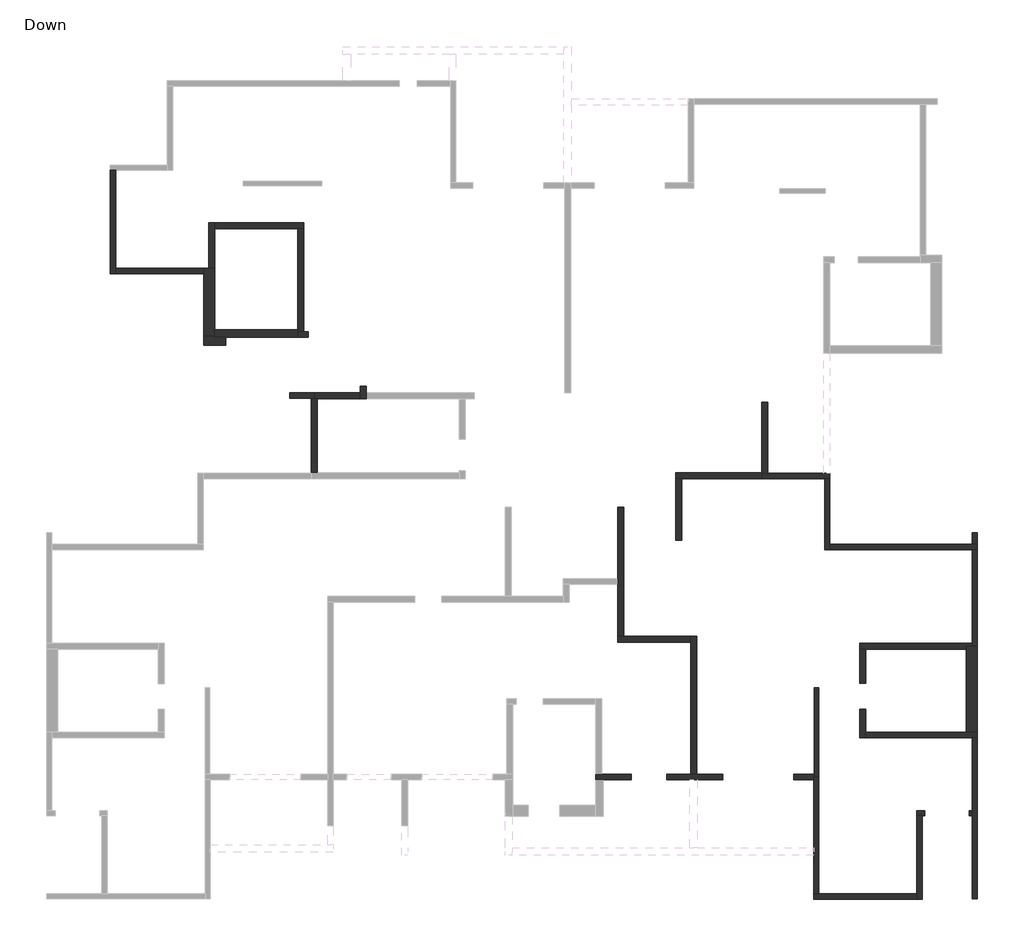
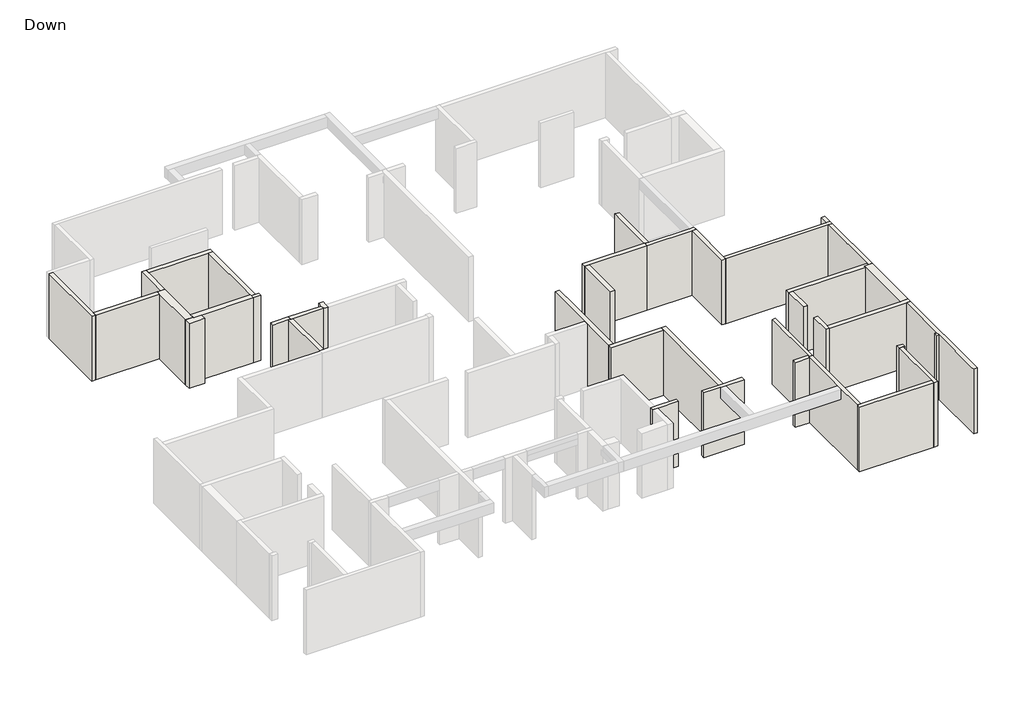
# One storey, part 2 of 3: 39 walls.
"""IFC4 building model written with IfcOpenShell, lengths in millimetres."""

from ifc_helpers import new_model, si_unit, origin, origin_with_axes, place, context, project, spatial, polyline, outline, extrude, faceted_brep, element, save

model = new_model("IFC4")

# Units and contexts
model_context = context("Model", 3, world=origin())
ifc_project = project(units=[si_unit("LENGTHUNIT", "METRE", prefix="MILLI")], contexts=[model_context])

# Site, building, storey
site = spatial("IfcSite", under=ifc_project)
building = spatial("IfcBuilding", under=site)
storey = spatial("IfcBuildingStorey", under=building, Name="Down", Elevation=0.0)

# Walls
placement = place(None, origin())
element("IfcWall", 1, ObjectType="15", at=placement, inside=storey, context=model_context, shape_type="Brep", body=[
    faceted_brep([(7365.3434642, -11434.051338, 0.0), (7365.3434642, -8419.051338, 0.0), (7365.3434642, -8419.051338, 3000.0), (7365.3434642, -8419.051338, 3200.0), (7365.3434642, -11434.051338, 3200.0), (7215.3434642, -11434.051338, 0.0), (7215.3434642, -11434.051338, 3200.0), (7215.3434642, -11344.051338, 3200.0), (7215.3434642, -8419.051338, 3200.0), (7215.3434642, -8419.051338, 3000.0), (7215.3434642, -8419.051338, 0.0), (7215.3434642, -11344.051338, 0.0)], [[[0, 1, 2, 3, 4]], [[5, 6, 7, 8, 9, 10, 11]], [[1, 0, 5, 11, 10]], [[3, 2, 1, 10, 9, 8]], [[4, 3, 8, 7, 6]], [[0, 4, 6, 5]]]),
])
element("IfcWall", 2, ObjectType="18", at=placement, inside=storey, context=model_context, shape_type="Brep", body=[
    faceted_brep([(-16547.4366188, 9037.0772927, 0.0), (-16547.4366188, 5556.9611102, 0.0), (-16547.4366188, 5556.9611102, 3200.0), (-16547.4366188, 9037.0772927, 3200.0), (-16367.4366188, 9037.0772927, 0.0), (-16367.4366188, 9037.0772927, 3000.0), (-16367.4366188, 9037.0772927, 3200.0), (-16367.4366188, 5736.9611102, 3200.0), (-16367.4366188, 5556.9611102, 3200.0), (-16367.4366188, 5556.9611102, 0.0), (-16367.4366188, 5736.9611102, 0.0)], [[[0, 1, 2, 3]], [[4, 5, 6, 7, 8, 9, 10]], [[1, 0, 4, 10, 9]], [[3, 2, 8, 7, 6]], [[0, 3, 6, 5, 4]], [[2, 1, 9, 8]]]),
])
element("IfcWall", 3, ObjectType="18", at=placement, inside=storey, context=model_context, shape_type="Brep", body=[
    faceted_brep([(-16367.4366188, 5556.9611102, 0.0), (-13386.7312246, 5556.9611102, 0.0), (-13386.7312246, 5556.9611102, 3200.0), (-16367.4366188, 5556.9611102, 3200.0), (-16367.4366188, 5736.9611102, 0.0), (-16367.4366188, 5736.9611102, 3000.0), (-16367.4366188, 5736.9611102, 3200.0), (-13386.7312246, 5736.9611102, 3200.0), (-13386.7312246, 5736.9611102, 0.0)], [[[0, 1, 2, 3]], [[4, 5, 6, 7, 8]], [[1, 0, 4, 8]], [[3, 2, 7, 6]], [[0, 3, 6, 5, 4]], [[2, 1, 8, 7]]]),
])
element("IfcWall", 4, ObjectType="18", at=placement, inside=storey, context=model_context, shape_type="Brep", body=[
    faceted_brep([(-10217.2125524, 3416.4548861, 0.0), (-9872.2125524, 3416.4548861, 0.0), (-9872.2125524, 3416.4548861, 3000.0), (-9872.2125524, 3416.4548861, 3200.0), (-10217.2125524, 3416.4548861, 3200.0), (-10217.2125524, 3596.4548861, 0.0), (-10217.2125524, 3596.4548861, 3200.0), (-10017.2125524, 3596.4548861, 3200.0), (-9872.2125524, 3596.4548861, 3200.0), (-9872.2125524, 3596.4548861, 3000.0), (-9872.2125524, 3596.4548861, 0.0), (-10017.2125524, 3596.4548861, 0.0)], [[[0, 1, 2, 3, 4]], [[5, 6, 7, 8, 9, 10, 11]], [[1, 0, 5, 11, 10]], [[3, 2, 1, 10, 9, 8]], [[4, 3, 8, 7, 6]], [[0, 4, 6, 5]]]),
])
element("IfcWall", 5, ObjectType="18", at=placement, inside=storey, context=model_context, shape_type="Brep", body=[
    faceted_brep([(7735.384958, -1184.051338, 0.0), (5633.824792, -1184.051338, 0.0), (5433.824792, -1184.051338, 0.0), (5433.824792, -1184.051338, 3200.0), (5633.824792, -1184.051338, 3200.0), (7535.1359953, -1184.051338, 3200.0), (7735.384958, -1184.051338, 3200.0), (7735.384958, -1364.051338, 0.0), (7735.384958, -1364.051338, 3200.0), (7555.384958, -1364.051338, 3200.0), (5433.824792, -1364.051338, 3200.0), (5433.824792, -1364.051338, 0.0), (7555.384958, -1364.051338, 0.0)], [[[0, 1, 2, 3, 4, 5, 6]], [[7, 8, 9, 10, 11, 12]], [[2, 1, 0, 7, 12, 11]], [[6, 5, 4, 3, 10, 9, 8]], [[3, 2, 11, 10]], [[0, 6, 8, 7]]]),
])
element("IfcWall", 6, ObjectType="18", at=placement, inside=storey, context=model_context, shape_type="Brep", body=[
    faceted_brep([(7555.384958, -1364.051338, 0.0), (7555.384958, -3764.1011305, 0.0), (7555.384958, -3764.1011305, 3000.0), (7555.384958, -3764.1011305, 3200.0), (7555.384958, -1364.051338, 3200.0), (7555.384958, -1364.051338, 3000.0), (7735.384958, -1364.051338, 0.0), (7735.384958, -1364.051338, 3200.0), (7735.384958, -3584.1011305, 3200.0), (7735.384958, -3764.1011305, 3200.0), (7735.384958, -3764.1011305, 0.0), (7735.384958, -3584.1011305, 0.0)], [[[0, 1, 2, 3, 4, 5]], [[6, 7, 8, 9, 10, 11]], [[1, 0, 6, 11, 10]], [[4, 3, 9, 8, 7]], [[3, 2, 1, 10, 9]], [[0, 5, 4, 7, 6]]]),
])
element("IfcWall", 7, ObjectType="18", at=placement, inside=storey, context=model_context, shape_type="Brep", body=[
    faceted_brep([(7735.384958, -3764.1011305, 0.0), (12534.2065347, -3764.1011305, 0.0), (12714.2065347, -3764.1011305, 0.0), (12714.2065347, -3764.1011305, 3200.0), (12534.2065347, -3764.1011305, 3200.0), (7735.384958, -3764.1011305, 3200.0), (7735.384958, -3584.1011305, 0.0), (7735.384958, -3584.1011305, 3200.0), (12534.2065347, -3584.1011305, 3200.0), (12714.2065347, -3584.1011305, 3200.0), (12714.2065347, -3584.1011305, 0.0), (12534.2065347, -3584.1011305, 0.0)], [[[0, 1, 2, 3, 4, 5]], [[6, 7, 8, 9, 10, 11]], [[2, 1, 0, 6, 11, 10]], [[5, 4, 3, 9, 8, 7]], [[0, 5, 7, 6]], [[3, 2, 10, 9]]]),
])
element("IfcWall", 8, ObjectType="18", at=placement, inside=storey, context=model_context, shape_type="SweptSolid", body=[
    extrude(outline(polyline([(12714.2065347, -3184.4330807), (12714.2065347, -3584.1011305), (12534.2065347, -3584.1011305), (12534.2065347, -3184.4330807), (12714.2065347, -3184.4330807)])), origin_with_axes(), (0.0, 0.0, 1.0), 3200.0),
])
element("IfcWall", 9, ObjectType="18", at=placement, inside=storey, context=model_context, shape_type="Brep", body=[
    faceted_brep([(12534.2065347, -3764.1011305, 0.0), (12534.2065347, -6913.2795537, 0.0), (12534.2065347, -7013.2795537, 0.0), (12534.2065347, -7013.2795537, 3200.0), (12534.2065347, -6913.2795537, 3200.0), (12534.2065347, -3764.1011305, 3200.0), (12534.2065347, -3764.1011305, 3000.0), (12714.2065347, -3764.1011305, 0.0), (12714.2065347, -3764.1011305, 3200.0), (12714.2065347, -7013.2795537, 3200.0), (12714.2065347, -7013.2795537, 0.0)], [[[0, 1, 2, 3, 4, 5, 6]], [[7, 8, 9, 10]], [[2, 1, 0, 7, 10]], [[3, 2, 10, 9]], [[5, 4, 3, 9, 8]], [[0, 6, 5, 8, 7]]]),
])
element("IfcWall", 10, ObjectType="18", at=placement, inside=storey, context=model_context, shape_type="Brep", body=[
    faceted_brep([(12534.2065347, -10113.0471886, 0.0), (12534.2065347, -12564.5160683, 0.0), (12534.2065347, -12744.5160683, 0.0), (12534.2065347, -15545.0637861, 0.0), (12534.2065347, -15545.0637861, 3200.0), (12534.2065347, -15369.5160683, 3200.0), (12534.2065347, -12744.5160683, 3200.0), (12534.2065347, -12564.5160683, 3200.0), (12534.2065347, -10113.0471886, 3200.0), (12534.2065347, -10113.0471886, 3000.0), (12714.2065347, -10113.0471886, 0.0), (12714.2065347, -10113.0471886, 3200.0), (12714.2065347, -15545.0637861, 3200.0), (12714.2065347, -15545.0637861, 0.0)], [[[0, 1, 2, 3, 4, 5, 6, 7, 8, 9]], [[10, 11, 12, 13]], [[3, 2, 1, 0, 10, 13]], [[4, 3, 13, 12]], [[8, 7, 6, 5, 4, 12, 11]], [[0, 9, 8, 11, 10]]]),
])
element("IfcWall", 11, ObjectType="18", at=placement, inside=storey, context=model_context, shape_type="Brep", body=[
    faceted_brep([(12534.2065347, -12564.5160683, 0.0), (12429.6422194, -12564.5160683, 0.0), (12429.6422194, -12564.5160683, 3000.0), (12429.6422194, -12564.5160683, 3200.0), (12534.2065347, -12564.5160683, 3200.0), (12534.2065347, -12564.5160683, 3000.0), (12534.2065347, -12744.5160683, 0.0), (12534.2065347, -12744.5160683, 2980.0), (12534.2065347, -12744.5160683, 3200.0), (12429.6422194, -12744.5160683, 3200.0), (12429.6422194, -12744.5160683, 3000.0), (12429.6422194, -12744.5160683, 0.0)], [[[0, 1, 2, 3, 4, 5]], [[6, 7, 8, 9, 10, 11]], [[1, 0, 6, 11]], [[3, 2, 1, 11, 10, 9]], [[4, 3, 9, 8]], [[0, 5, 4, 8, 7, 6]]]),
])
element("IfcWall", 12, ObjectType="18", at=placement, inside=storey, context=model_context, shape_type="Brep", body=[
    faceted_brep([(10930.9368252, -12564.5160683, 0.0), (10665.3434642, -12564.5160683, 0.0), (10665.3434642, -12564.5160683, 3000.0), (10665.3434642, -12564.5160683, 3200.0), (10930.9368252, -12564.5160683, 3200.0), (10930.9368252, -12564.5160683, 3000.0), (10930.9368252, -12744.5160683, 0.0), (10930.9368252, -12744.5160683, 3000.0), (10930.9368252, -12744.5160683, 3200.0), (10845.3434642, -12744.5160683, 3200.0), (10665.3434642, -12744.5160683, 3200.0), (10665.3434642, -12744.5160683, 0.0), (10845.3434642, -12744.5160683, 0.0)], [[[0, 1, 2, 3, 4, 5]], [[6, 7, 8, 9, 10, 11, 12]], [[1, 0, 6, 12, 11]], [[4, 3, 10, 9, 8]], [[0, 5, 4, 8, 7, 6]], [[3, 2, 1, 11, 10]]]),
])
element("IfcWall", 13, ObjectType="18", at=placement, inside=storey, context=model_context, shape_type="Brep", body=[
    faceted_brep([(10665.3434642, -12744.5160683, 0.0), (10665.3434642, -15369.5160683, 0.0), (10665.3434642, -15549.5160683, 0.0), (10665.3434642, -15549.5160683, 3200.0), (10665.3434642, -15369.5160683, 3200.0), (10665.3434642, -12744.5160683, 3200.0), (10845.3434642, -12744.5160683, 0.0), (10845.3434642, -12744.5160683, 2980.0), (10845.3434642, -12744.5160683, 3200.0), (10845.3434642, -15369.5160683, 3200.0), (10845.3434642, -15549.5160683, 3200.0), (10845.3434642, -15549.5160683, 0.0)], [[[0, 1, 2, 3, 4, 5]], [[6, 7, 8, 9, 10, 11]], [[2, 1, 0, 6, 11]], [[5, 4, 3, 10, 9, 8]], [[0, 5, 8, 7, 6]], [[3, 2, 11, 10]]]),
])
element("IfcWall", 14, ObjectType="18", at=placement, inside=storey, context=model_context, shape_type="Brep", body=[
    faceted_brep([(10665.3434642, -15369.5160683, 0.0), (7365.3434642, -15369.5160683, 0.0), (7185.3434642, -15369.5160683, 0.0), (7185.3434642, -15369.5160683, 3200.0), (7365.3434642, -15369.5160683, 3200.0), (10665.3434642, -15369.5160683, 3200.0), (10665.3434642, -15369.5160683, 3000.0), (10665.3434642, -15549.5160683, 0.0), (10665.3434642, -15549.5160683, 3200.0), (7185.3434642, -15549.5160683, 3200.0), (7185.3434642, -15549.5160683, 0.0)], [[[0, 1, 2, 3, 4, 5, 6]], [[7, 8, 9, 10]], [[2, 1, 0, 7, 10]], [[5, 4, 3, 9, 8]], [[0, 6, 5, 8, 7]], [[3, 2, 10, 9]]]),
])
element("IfcWall", 15, ObjectType="18", at=placement, inside=storey, context=model_context, shape_type="Brep", body=[
    faceted_brep([(7365.3434642, -15369.5160683, 0.0), (7365.3434642, -11434.051338, 0.0), (7365.3434642, -11434.051338, 3200.0), (7365.3434642, -15369.5160683, 3200.0), (7365.3434642, -15369.5160683, 3000.0), (7185.3434642, -15369.5160683, 0.0), (7185.3434642, -15369.5160683, 3200.0), (7185.3434642, -13814.491172, 3200.0), (7185.3434642, -11524.051338, 3200.0), (7185.3434642, -11434.051338, 3200.0), (7185.3434642, -11434.051338, 0.0), (7185.3434642, -11524.051338, 0.0), (7215.3434642, -11434.051338, 0.0), (7215.3434642, -11434.051338, 3200.0)], [[[0, 1, 2, 3, 4]], [[5, 6, 7, 8, 9, 10, 11]], [[1, 0, 5, 11, 10, 12]], [[2, 1, 12, 10, 9, 13]], [[3, 2, 13, 9, 8, 7, 6]], [[0, 4, 3, 6, 5]]]),
])
element("IfcWall", 16, ObjectType="18", at=placement, inside=storey, context=model_context, shape_type="Brep", body=[
    faceted_brep([(7215.3434642, -11344.051338, 0.0), (6514.9202277, -11344.051338, 0.0), (6514.9202277, -11344.051338, 3000.0), (6514.9202277, -11344.051338, 3200.0), (7215.3434642, -11344.051338, 3200.0), (7215.3434642, -11344.051338, 3000.0), (7185.3434642, -11524.051338, 0.0), (7185.3434642, -11524.051338, 2980.0), (7185.3434642, -11524.051338, 3200.0), (6514.9202277, -11524.051338, 3200.0), (6514.9202277, -11524.051338, 3000.0), (6514.9202277, -11524.051338, 0.0), (7215.3434642, -11434.051338, 0.0), (7185.3434642, -11434.051338, 0.0), (7185.3434642, -11434.051338, 3200.0), (7215.3434642, -11434.051338, 3200.0)], [[[0, 1, 2, 3, 4, 5]], [[6, 7, 8, 9, 10, 11]], [[1, 0, 12, 13, 6, 11]], [[3, 2, 1, 11, 10, 9]], [[4, 3, 9, 8, 14, 15]], [[0, 5, 4, 15, 12]], [[15, 14, 13, 12]], [[14, 8, 7, 6, 13]]]),
])
element("IfcWall", 17, ObjectType="18", at=placement, inside=storey, context=model_context, shape_type="Brep", body=[
    faceted_brep([(4114.0405596, -11344.051338, 0.0), (3235.0530078, -11344.051338, 0.0), (3035.0530078, -11344.051338, 0.0), (2233.8081945, -11344.051338, 0.0), (2233.8081945, -11344.051338, 3000.0), (2233.8081945, -11344.051338, 3200.0), (3035.0530078, -11344.051338, 3200.0), (3235.0530078, -11344.051338, 3200.0), (4114.0405596, -11344.051338, 3200.0), (4114.0405596, -11344.051338, 3000.0), (4114.0405596, -11524.051338, 0.0), (4114.0405596, -11524.051338, 3000.0), (4114.0405596, -11524.051338, 3200.0), (3265.0530078, -11524.051338, 3200.0), (2233.8081945, -11524.051338, 3200.0), (2233.8081945, -11524.051338, 3000.0), (2233.8081945, -11524.051338, 0.0)], [[[0, 1, 2, 3, 4, 5, 6, 7, 8, 9]], [[10, 11, 12, 13, 14, 15, 16]], [[3, 2, 1, 0, 10, 16]], [[5, 4, 3, 16, 15, 14]], [[8, 7, 6, 5, 14, 13, 12]], [[0, 9, 8, 12, 11, 10]]]),
])
element("IfcWall", 18, ObjectType="18", at=placement, inside=storey, context=model_context, shape_type="Brep", body=[
    faceted_brep([(1034.4223024, -11344.051338, 0.0), (35.0364103, -11344.051338, 0.0), (-164.9635897, -11344.051338, 0.0), (-164.9635897, -11344.051338, 3200.0), (35.0364103, -11344.051338, 3200.0), (1034.4223024, -11344.051338, 3200.0), (1034.4223024, -11344.051338, 3000.0), (1034.4223024, -11524.051338, 0.0), (1034.4223024, -11524.051338, 3000.0), (1034.4223024, -11524.051338, 3200.0), (85.0364103, -11524.051338, 3200.0), (-164.9635897, -11524.051338, 3200.0), (-164.9635897, -11524.051338, 0.0), (85.0364103, -11524.051338, 0.0)], [[[0, 1, 2, 3, 4, 5, 6]], [[7, 8, 9, 10, 11, 12, 13]], [[2, 1, 0, 7, 13, 12]], [[5, 4, 3, 11, 10, 9]], [[0, 6, 5, 9, 8, 7]], [[3, 2, 12, 11]]]),
])
element("IfcWall", 19, ObjectType="18", at=placement, inside=storey, context=model_context, shape_type="Brep", body=[
    faceted_brep([(-9666.1254155, 1536.9777077, 0.0), (-10496.1254155, 1536.9777077, 0.0), (-10496.1254155, 1536.9777077, 3200.0), (-10356.1254155, 1536.9777077, 3200.0), (-9666.1254155, 1536.9777077, 3200.0), (-9666.1254155, 1356.9777077, 0.0), (-9666.1254155, 1356.9777077, 3200.0), (-9766.1254155, 1356.9777077, 3200.0), (-10496.1254155, 1356.9777077, 3200.0), (-10496.1254155, 1356.9777077, 0.0), (-9766.1254155, 1356.9777077, 0.0)], [[[0, 1, 2, 3, 4]], [[5, 6, 7, 8, 9, 10]], [[1, 0, 5, 10, 9]], [[2, 1, 9, 8]], [[4, 3, 2, 8, 7, 6]], [[0, 4, 6, 5]]]),
])
element("IfcWall", 20, ObjectType="20", at=placement, inside=storey, context=model_context, shape_type="Brep", body=[
    faceted_brep([(-13016.7312246, 5736.9611102, 0.0), (-13016.7312246, 7066.4548861, 0.0), (-13016.7312246, 7266.4548861, 0.0), (-13016.7312246, 7266.4548861, 3200.0), (-13016.7312246, 7066.4548861, 3200.0), (-13016.7312246, 5736.9611102, 3200.0), (-13216.7312246, 5736.9611102, 0.0), (-13216.7312246, 5736.9611102, 3000.0), (-13216.7312246, 5736.9611102, 3200.0), (-13216.7312246, 7266.4548861, 3200.0), (-13216.7312246, 7266.4548861, 3000.0), (-13216.7312246, 7266.4548861, 0.0)], [[[0, 1, 2, 3, 4, 5]], [[6, 7, 8, 9, 10, 11]], [[2, 1, 0, 6, 11]], [[5, 4, 3, 9, 8]], [[3, 2, 11, 10, 9]], [[0, 5, 8, 7, 6]]]),
])
element("IfcWall", 21, ObjectType="20", at=placement, inside=storey, context=model_context, shape_type="Brep", body=[
    faceted_brep([(-13016.7312246, 7066.4548861, 0.0), (-10217.2125524, 7066.4548861, 0.0), (-10017.2125524, 7066.4548861, 0.0), (-10017.2125524, 7066.4548861, 3200.0), (-10217.2125524, 7066.4548861, 3200.0), (-13016.7312246, 7066.4548861, 3200.0), (-13016.7312246, 7066.4548861, 3000.0), (-13016.7312246, 7266.4548861, 0.0), (-13016.7312246, 7266.4548861, 3200.0), (-10017.2125524, 7266.4548861, 3200.0), (-10017.2125524, 7266.4548861, 3000.0), (-10017.2125524, 7266.4548861, 0.0)], [[[0, 1, 2, 3, 4, 5, 6]], [[7, 8, 9, 10, 11]], [[2, 1, 0, 7, 11]], [[5, 4, 3, 9, 8]], [[0, 6, 5, 8, 7]], [[3, 2, 11, 10, 9]]]),
])
element("IfcWall", 22, ObjectType="20", at=placement, inside=storey, context=model_context, shape_type="Brep", body=[
    faceted_brep([(-10217.2125524, 7066.4548861, 0.0), (-10217.2125524, 3666.4548861, 0.0), (-10217.2125524, 3596.4548861, 0.0), (-10217.2125524, 3596.4548861, 3200.0), (-10217.2125524, 3666.4548861, 3200.0), (-10217.2125524, 7066.4548861, 3200.0), (-10217.2125524, 7066.4548861, 3000.0), (-10017.2125524, 7066.4548861, 0.0), (-10017.2125524, 7066.4548861, 3200.0), (-10017.2125524, 3596.4548861, 3200.0), (-10017.2125524, 3596.4548861, 3000.0), (-10017.2125524, 3596.4548861, 0.0)], [[[0, 1, 2, 3, 4, 5, 6]], [[7, 8, 9, 10, 11]], [[2, 1, 0, 7, 11]], [[5, 4, 3, 9, 8]], [[0, 6, 5, 8, 7]], [[3, 2, 11, 10, 9]]]),
])
element("IfcWall", 23, ObjectType="20", at=placement, inside=storey, context=model_context, shape_type="Brep", body=[
    faceted_brep([(5433.824792, 1223.1519815, 0.0), (5433.824792, -1164.051338, 0.0), (5433.824792, -1184.051338, 0.0), (5433.824792, -1184.051338, 3200.0), (5433.824792, -1164.051338, 3200.0), (5433.824792, 1223.1519815, 3200.0), (5433.824792, 1223.1519815, 3000.0), (5633.824792, 1223.1519815, 0.0), (5633.824792, 1223.1519815, 3000.0), (5633.824792, 1223.1519815, 3200.0), (5633.824792, -1184.051338, 3200.0), (5633.824792, -1184.051338, 3000.0), (5633.824792, -1184.051338, 0.0)], [[[0, 1, 2, 3, 4, 5, 6]], [[7, 8, 9, 10, 11, 12]], [[2, 1, 0, 7, 12]], [[5, 4, 3, 10, 9]], [[0, 6, 5, 9, 8, 7]], [[3, 2, 12, 11, 10]]]),
])
element("IfcWall", 24, ObjectType="20", at=placement, inside=storey, context=model_context, shape_type="Brep", body=[
    faceted_brep([(5433.824792, -1164.051338, 0.0), (2535.2355804, -1164.051338, 0.0), (2535.2355804, -1164.051338, 3000.0), (2535.2355804, -1164.051338, 3200.0), (5433.824792, -1164.051338, 3200.0), (5433.824792, -1164.051338, 3000.0), (5433.824792, -1364.051338, 0.0), (5433.824792, -1364.051338, 3200.0), (2735.2355804, -1364.051338, 3200.0), (2535.2355804, -1364.051338, 3200.0), (2535.2355804, -1364.051338, 0.0), (2735.2355804, -1364.051338, 0.0), (5433.824792, -1184.051338, 0.0), (5433.824792, -1184.051338, 3200.0)], [[[0, 1, 2, 3, 4, 5]], [[6, 7, 8, 9, 10, 11]], [[1, 0, 12, 6, 11, 10]], [[4, 3, 9, 8, 7, 13]], [[0, 5, 4, 13, 7, 6, 12]], [[3, 2, 1, 10, 9]]]),
])
element("IfcWall", 25, ObjectType="20", at=placement, inside=storey, context=model_context, shape_type="Brep", body=[
    faceted_brep([(2535.2355804, -1364.051338, 0.0), (2535.2355804, -3433.1633712, 0.0), (2535.2355804, -3433.1633712, 3000.0), (2535.2355804, -3433.1633712, 3200.0), (2535.2355804, -1364.051338, 3200.0), (2735.2355804, -1364.051338, 0.0), (2735.2355804, -1364.051338, 3000.0), (2735.2355804, -1364.051338, 3200.0), (2735.2355804, -3433.1633712, 3200.0), (2735.2355804, -3433.1633712, 3000.0), (2735.2355804, -3433.1633712, 0.0)], [[[0, 1, 2, 3, 4]], [[5, 6, 7, 8, 9, 10]], [[1, 0, 5, 10]], [[3, 2, 1, 10, 9, 8]], [[4, 3, 8, 7]], [[0, 4, 7, 6, 5]]]),
])
element("IfcWall", 26, ObjectType="20", at=placement, inside=storey, context=model_context, shape_type="Brep", body=[
    faceted_brep([(12534.2065347, -6913.2795537, 0.0), (8750.0364103, -6913.2795537, 0.0), (8750.0364103, -6913.2795537, 3000.0), (8750.0364103, -6913.2795537, 3200.0), (12534.2065347, -6913.2795537, 3200.0), (12534.2065347, -6913.2795537, 3000.0), (12344.2065347, -7113.2795537, 0.0), (12344.2065347, -7113.2795537, 3000.0), (12344.2065347, -7113.2795537, 3200.0), (8950.0364103, -7113.2795537, 3200.0), (8750.0364103, -7113.2795537, 3200.0), (8750.0364103, -7113.2795537, 0.0), (8950.0364103, -7113.2795537, 0.0), (12534.2065347, -7013.2795537, 0.0), (12344.2065347, -7013.2795537, 0.0), (12344.2065347, -7013.2795537, 3200.0), (12534.2065347, -7013.2795537, 3200.0)], [[[0, 1, 2, 3, 4, 5]], [[6, 7, 8, 9, 10, 11, 12]], [[1, 0, 13, 14, 6, 12, 11]], [[4, 3, 10, 9, 8, 15, 16]], [[3, 2, 1, 11, 10]], [[0, 5, 4, 16, 13]], [[16, 15, 14, 13]], [[15, 8, 7, 6, 14]]]),
])
element("IfcWall", 27, ObjectType="20", at=placement, inside=storey, context=model_context, shape_type="Brep", body=[
    faceted_brep([(8750.0364103, -7113.2795537, 0.0), (8750.0364103, -8273.2795537, 0.0), (8750.0364103, -8273.2795537, 3000.0), (8750.0364103, -8273.2795537, 3200.0), (8750.0364103, -7113.2795537, 3200.0), (8950.0364103, -7113.2795537, 0.0), (8950.0364103, -7113.2795537, 3000.0), (8950.0364103, -7113.2795537, 3200.0), (8950.0364103, -8273.2795537, 3200.0), (8950.0364103, -8273.2795537, 3000.0), (8950.0364103, -8273.2795537, 0.0), (8945.0613065, -8273.2795537, 3200.0)], [[[0, 1, 2, 3, 4]], [[5, 6, 7, 8, 9, 10]], [[1, 0, 5, 10]], [[3, 2, 1, 10, 9, 8, 11]], [[4, 3, 11, 8, 7]], [[0, 4, 7, 6, 5]]]),
])
element("IfcWall", 28, ObjectType="20", at=placement, inside=storey, context=model_context, shape_type="Brep", body=[
    faceted_brep([(8745.0613065, -9149.744284, 0.0), (8745.0613065, -10113.0471886, 0.0), (8745.0613065, -10113.0471886, 3000.0), (8745.0613065, -10113.0471886, 3200.0), (8745.0613065, -9149.744284, 3200.0), (8745.0613065, -9149.744284, 3000.0), (8945.0613065, -9149.744284, 0.0), (8945.0613065, -9149.744284, 3000.0), (8945.0613065, -9149.744284, 3200.0), (8945.0613065, -9913.0471886, 3200.0), (8945.0613065, -10113.0471886, 3200.0), (8945.0613065, -10113.0471886, 0.0), (8945.0613065, -9913.0471886, 0.0)], [[[0, 1, 2, 3, 4, 5]], [[6, 7, 8, 9, 10, 11, 12]], [[1, 0, 6, 12, 11]], [[4, 3, 10, 9, 8]], [[0, 5, 4, 8, 7, 6]], [[3, 2, 1, 11, 10]]]),
])
element("IfcWall", 29, ObjectType="20", at=placement, inside=storey, context=model_context, shape_type="Brep", body=[
    faceted_brep([(8945.0613065, -10113.0471886, 0.0), (12534.2065347, -10113.0471886, 0.0), (12714.2065347, -10113.0471886, 0.0), (12714.2065347, -10113.0471886, 3200.0), (12534.2065347, -10113.0471886, 3200.0), (8945.0613065, -10113.0471886, 3200.0), (8945.0613065, -9913.0471886, 0.0), (8945.0613065, -9913.0471886, 3000.0), (8945.0613065, -9913.0471886, 3200.0), (12344.2065347, -9913.0471886, 3200.0), (12714.2065347, -9913.0471886, 3200.0), (12714.2065347, -9913.0471886, 0.0), (12344.2065347, -9913.0471886, 0.0)], [[[0, 1, 2, 3, 4, 5]], [[6, 7, 8, 9, 10, 11, 12]], [[2, 1, 0, 6, 12, 11]], [[5, 4, 3, 10, 9, 8]], [[0, 5, 8, 7, 6]], [[3, 2, 11, 10]]]),
])
element("IfcWall", 30, ObjectType="20", at=placement, inside=storey, context=model_context, shape_type="Brep", body=[
    faceted_brep([(3235.0530078, -11344.051338, 0.0), (3235.0530078, -6683.5202176, 0.0), (3235.0530078, -6683.5202176, 3000.0), (3235.0530078, -6683.5202176, 3200.0), (3235.0530078, -11344.051338, 3200.0), (3235.0530078, -11344.051338, 3000.0), (3035.0530078, -11344.051338, 0.0), (3035.0530078, -11344.051338, 3000.0), (3035.0530078, -11344.051338, 3200.0), (3035.0530078, -6883.5202176, 3200.0), (3035.0530078, -6683.5202176, 3200.0), (3035.0530078, -6683.5202176, 0.0), (3035.0530078, -6883.5202176, 0.0)], [[[0, 1, 2, 3, 4, 5]], [[6, 7, 8, 9, 10, 11, 12]], [[1, 0, 6, 12, 11]], [[4, 3, 10, 9, 8]], [[0, 5, 4, 8, 7, 6]], [[3, 2, 1, 11, 10]]]),
])
element("IfcWall", 31, ObjectType="20", at=placement, inside=storey, context=model_context, shape_type="Brep", body=[
    faceted_brep([(3035.0530078, -6683.5202176, 0.0), (783.3351654, -6683.5202176, 0.0), (583.3351654, -6683.5202176, 0.0), (583.3351654, -6683.5202176, 3200.0), (783.3351654, -6683.5202176, 3200.0), (3035.0530078, -6683.5202176, 3200.0), (3035.0530078, -6883.5202176, 0.0), (3035.0530078, -6883.5202176, 3000.0), (3035.0530078, -6883.5202176, 3200.0), (583.3351654, -6883.5202176, 3200.0), (583.3351654, -6883.5202176, 3000.0), (583.3351654, -6883.5202176, 0.0)], [[[0, 1, 2, 3, 4, 5]], [[6, 7, 8, 9, 10, 11]], [[2, 1, 0, 6, 11]], [[5, 4, 3, 9, 8]], [[0, 5, 8, 7, 6]], [[3, 2, 11, 10, 9]]]),
])
element("IfcWall", 32, ObjectType="20", at=placement, inside=storey, context=model_context, shape_type="Brep", body=[
    faceted_brep([(783.3351654, -6683.5202176, 0.0), (783.3351654, -2332.8480185, 0.0), (783.3351654, -2332.8480185, 3000.0), (783.3351654, -2332.8480185, 3200.0), (783.3351654, -3433.1633712, 3200.0), (783.3351654, -6683.5202176, 3200.0), (783.3351654, -6683.5202176, 3000.0), (583.3351654, -6683.5202176, 0.0), (583.3351654, -6683.5202176, 3200.0), (583.3351654, -4933.7276865, 3200.0), (583.3351654, -4733.7276865, 3200.0), (583.3351654, -2332.8480185, 3200.0), (583.3351654, -2332.8480185, 0.0), (583.3351654, -4733.7276865, 0.0), (583.3351654, -4933.7276865, 0.0)], [[[0, 1, 2, 3, 4, 5, 6]], [[7, 8, 9, 10, 11, 12, 13, 14]], [[1, 0, 7, 14, 13, 12]], [[3, 2, 1, 12, 11]], [[5, 4, 3, 11, 10, 9, 8]], [[0, 6, 5, 8, 7]]]),
])
element("IfcWall", 33, ObjectType="20", at=placement, inside=storey, context=model_context, shape_type="Brep", body=[
    faceted_brep([(-7916.2250005, 1337.2266703, 0.0), (-7916.2250005, 1537.2266703, 0.0), (-7916.2250005, 1752.2266703, 0.0), (-7916.2250005, 1752.2266703, 3000.0), (-7916.2250005, 1752.2266703, 3200.0), (-7916.2250005, 1537.2266703, 3200.0), (-7916.2250005, 1337.2266703, 3200.0), (-8116.2250005, 1337.2266703, 0.0), (-8116.2250005, 1337.2266703, 3200.0), (-8116.2250005, 1536.9777077, 3200.0), (-8116.2250005, 1752.2266703, 3200.0), (-8116.2250005, 1752.2266703, 3000.0), (-8116.2250005, 1752.2266703, 0.0), (-8116.2250005, 1536.9777077, 0.0)], [[[0, 1, 2, 3, 4, 5, 6]], [[7, 8, 9, 10, 11, 12, 13]], [[2, 1, 0, 7, 13, 12]], [[4, 3, 2, 12, 11, 10]], [[6, 5, 4, 10, 9, 8]], [[0, 6, 8, 7]]]),
])
element("IfcWall", 34, ObjectType="20", at=placement, inside=storey, context=model_context, shape_type="Brep", body=[
    faceted_brep([(-8116.2250005, 1536.9777077, 0.0), (-9666.1254155, 1536.9777077, 0.0), (-9666.1254155, 1536.9777077, 3200.0), (-8116.2250005, 1536.9777077, 3200.0), (-8116.2250005, 1536.9777077, 3000.0), (-8116.2250005, 1336.9777077, 0.0), (-8116.2250005, 1336.9777077, 3200.0), (-9566.1254155, 1336.9777077, 3200.0), (-9666.1254155, 1336.9777077, 3200.0), (-9666.1254155, 1336.9777077, 0.0), (-9566.1254155, 1336.9777077, 0.0), (-8116.2250005, 1337.2266703, 0.0), (-9666.1254155, 1356.9777077, 0.0), (-9666.1254155, 1356.9777077, 3200.0), (-8116.2250005, 1337.2266703, 3200.0)], [[[0, 1, 2, 3, 4]], [[5, 6, 7, 8, 9, 10]], [[1, 0, 11, 5, 10, 9, 12]], [[2, 1, 12, 9, 8, 13]], [[3, 2, 13, 8, 7, 6, 14]], [[0, 4, 3, 14, 6, 5, 11]]]),
])
element("IfcWall", 35, ObjectType="20", at=placement, inside=storey, context=model_context, shape_type="SweptSolid", body=[
    extrude(outline(polyline([(-9766.1254155, -1164.051338), (-9766.1254155, 1356.9777077), (-9666.1254155, 1356.9777077), (-9666.1254155, 1336.9777077), (-9566.1254155, 1336.9777077), (-9566.1254155, -1164.051338), (-9766.1254155, -1164.051338)])), origin_with_axes(), (0.0, 0.0, 1.0), 3200.0),
])
element("IfcWall", 36, ObjectType="25", at=placement, inside=storey, context=model_context, shape_type="Brep", body=[
    faceted_brep([(-10217.2125524, 3666.4548861, 0.0), (-13016.7312246, 3666.4548861, 0.0), (-13016.7312246, 3666.4548861, 3000.0), (-13016.7312246, 3666.4548861, 3200.0), (-10217.2125524, 3666.4548861, 3200.0), (-10217.2125524, 3666.4548861, 3000.0), (-10217.2125524, 3416.4548861, 0.0), (-10217.2125524, 3416.4548861, 3200.0), (-10356.1254155, 3416.4548861, 3200.0), (-12647.8515565, 3416.4548861, 3200.0), (-13016.7312246, 3416.4548861, 3200.0), (-13016.7312246, 3416.4548861, 0.0), (-12647.8515565, 3416.4548861, 0.0), (-10217.2125524, 3596.4548861, 0.0), (-13016.7312246, 3445.542023, 0.0), (-13016.7312246, 3445.542023, 3200.0), (-10217.2125524, 3596.4548861, 3200.0)], [[[0, 1, 2, 3, 4, 5]], [[6, 7, 8, 9, 10, 11, 12]], [[1, 0, 13, 6, 12, 11, 14]], [[4, 3, 15, 10, 9, 8, 7, 16]], [[3, 2, 1, 14, 11, 10, 15]], [[0, 5, 4, 16, 7, 6, 13]]]),
])
element("IfcWall", 37, ObjectType="30", at=placement, inside=storey, context=model_context, shape_type="SweptSolid", body=[
    extrude(outline(polyline([(-12647.8515565, 3145.542023), (-13386.7312246, 3145.542023), (-13386.7312246, 3445.542023), (-13016.7312246, 3445.542023), (-13016.7312246, 3416.4548861), (-12647.8515565, 3416.4548861), (-12647.8515565, 3145.542023)])), origin_with_axes(), (0.0, 0.0, 1.0), 3200.0),
])
element("IfcWall", 38, ObjectType="37", at=placement, inside=storey, context=model_context, shape_type="Brep", body=[
    faceted_brep([(-13386.7312246, 5736.9611102, 0.0), (-13386.7312246, 5556.9611102, 0.0), (-13386.7312246, 3445.542023, 0.0), (-13386.7312246, 3445.542023, 3200.0), (-13386.7312246, 5556.9611102, 3200.0), (-13386.7312246, 5736.9611102, 3200.0), (-13016.7312246, 5736.9611102, 0.0), (-13016.7312246, 5736.9611102, 3200.0), (-13016.7312246, 3666.4548861, 3200.0), (-13016.7312246, 3445.542023, 3200.0), (-13016.7312246, 3445.542023, 0.0), (-13016.7312246, 3666.4548861, 0.0), (-13216.7312246, 5736.9611102, 0.0), (-13216.7312246, 5736.9611102, 3200.0)], [[[0, 1, 2, 3, 4, 5]], [[6, 7, 8, 9, 10, 11]], [[2, 1, 0, 12, 6, 11, 10]], [[5, 4, 3, 9, 8, 7, 13]], [[0, 5, 13, 7, 6, 12]], [[3, 2, 10, 9]]]),
])
element("IfcWall", 39, ObjectType="37", at=placement, inside=storey, context=model_context, shape_type="Brep", body=[
    faceted_brep([(12714.2065347, -9913.0471886, 0.0), (12714.2065347, -7013.2795537, 0.0), (12714.2065347, -7013.2795537, 3200.0), (12714.2065347, -9913.0471886, 3200.0), (12344.2065347, -7013.2795537, 3200.0), (12344.2065347, -7013.2795537, 0.0), (12344.2065347, -7113.2795537, 0.0), (12344.2065347, -9913.0471886, 0.0), (12344.2065347, -9913.0471886, 3000.0), (12344.2065347, -9913.0471886, 3200.0), (12344.2065347, -7113.2795537, 3200.0), (12534.2065347, -7013.2795537, 0.0), (12534.2065347, -7013.2795537, 3200.0)], [[[0, 1, 2, 3]], [[4, 5, 6, 7, 8, 9, 10]], [[1, 0, 7, 6, 5, 11]], [[2, 1, 11, 5, 4, 12]], [[3, 2, 12, 4, 10, 9]], [[0, 3, 9, 8, 7]]]),
])

save(model, "model.ifc")

# Revit data of these elements
# Type "15"
#   Layers, outside or top first: 15 cm "Concrete" (function 1)
# Type "18"
#   Layers, outside or top first: 18 cm "Concrete" (function 1)
# Type "20"
#   Layers, outside or top first: 20 cm "Concrete" (function 1)
# Type "25"
#   Layers, outside or top first: 25 cm "Concrete" (function 1)
# Type "30"
#   Layers, outside or top first: 30 cm "Concrete" (function 1)
# Type "37"
#   Layers, outside or top first: 37 cm "Concrete" (function 1)
# Element 1 (IfcWall, "15")
#   Comments = ""
#   Mark = "W99"
#   SOFiSTiK_EdgeZones = "W100"
#   SOFiSTiK_AMG_Comments = ""
#   Top Offset = 0 cm
#   Base Offset = 0 cm
#   wall height = 320 cm
#   SOFiSTiK_AMG_Scheduled = yes
#   SOFiSTiK_AMG_Adjusted = yes
#   Phase Created = New Construction
#   Base Constraint = Down
#   Top Constraint = Typical Floor
#   Materials on its faces: "Concrete"
# Element 2 (IfcWall, "18")
#   Comments = ""
#   Mark = "W48"
#   SOFiSTiK_EdgeZones = "W48"
#   SOFiSTiK_AMG_Comments = ""
#   Top Offset = 0 cm
#   Base Offset = 0 cm
#   wall height = 320 cm
#   SOFiSTiK_AMG_Scheduled = yes
#   SOFiSTiK_AMG_Adjusted = yes
#   Phase Created = New Construction
#   Base Constraint = Down
#   Top Constraint = Typical Floor
#   Materials on its faces: "Concrete"
# Element 3 (IfcWall, "18")
#   Comments = ""
#   Mark = "W49"
#   SOFiSTiK_EdgeZones = "W49"
#   SOFiSTiK_AMG_Comments = ""
#   Top Offset = 0 cm
#   Base Offset = 0 cm
#   wall height = 320 cm
#   SOFiSTiK_AMG_Scheduled = yes
#   SOFiSTiK_AMG_Adjusted = yes
#   Phase Created = New Construction
#   Base Constraint = Down
#   Top Constraint = Typical Floor
#   Materials on its faces: "Concrete"
# Element 4 (IfcWall, "18")
#   Comments = ""
#   Mark = "W50"
#   SOFiSTiK_EdgeZones = "W50"
#   SOFiSTiK_AMG_Comments = ""
#   Top Offset = 0 cm
#   Base Offset = 0 cm
#   wall height = 320 cm
#   SOFiSTiK_AMG_Scheduled = yes
#   SOFiSTiK_AMG_Adjusted = yes
#   Phase Created = New Construction
#   Base Constraint = Down
#   Top Constraint = Typical Floor
#   Materials on its faces: "Concrete"
# Element 5 (IfcWall, "18")
#   Comments = ""
#   Mark = "W55"
#   SOFiSTiK_EdgeZones = "W56"
#   SOFiSTiK_AMG_Comments = ""
#   Top Offset = 0 cm
#   Base Offset = 0 cm
#   wall height = 320 cm
#   SOFiSTiK_AMG_Scheduled = yes
#   SOFiSTiK_AMG_Adjusted = yes
#   Phase Created = New Construction
#   Base Constraint = Down
#   Top Constraint = Typical Floor
#   Materials on its faces: "Concrete"
# Element 6 (IfcWall, "18")
#   Comments = ""
#   Mark = "W56"
#   SOFiSTiK_EdgeZones = "W57"
#   SOFiSTiK_AMG_Comments = ""
#   Top Offset = 0 cm
#   Base Offset = 0 cm
#   wall height = 320 cm
#   SOFiSTiK_AMG_Scheduled = yes
#   SOFiSTiK_AMG_Adjusted = yes
#   Phase Created = New Construction
#   Base Constraint = Down
#   Top Constraint = Typical Floor
#   Materials on its faces: "Concrete"
# Element 7 (IfcWall, "18")
#   Comments = ""
#   Mark = "W57"
#   SOFiSTiK_EdgeZones = "W58"
#   SOFiSTiK_AMG_Comments = ""
#   Top Offset = 0 cm
#   Base Offset = 0 cm
#   wall height = 320 cm
#   SOFiSTiK_AMG_Scheduled = yes
#   SOFiSTiK_AMG_Adjusted = yes
#   Phase Created = New Construction
#   Base Constraint = Down
#   Top Constraint = Typical Floor
#   Materials on its faces: "Concrete"
# Element 8 (IfcWall, "18")
#   Comments = ""
#   Mark = "W58"
#   SOFiSTiK_EdgeZones = "W59"
#   SOFiSTiK_AMG_Comments = ""
#   Top Offset = 0 cm
#   Base Offset = 0 cm
#   wall height = 320 cm
#   SOFiSTiK_AMG_Scheduled = yes
#   SOFiSTiK_AMG_Adjusted = yes
#   Phase Created = New Construction
#   Base Constraint = Down
#   Top Constraint = Typical Floor
#   Materials on its faces: "Concrete"
# Element 9 (IfcWall, "18")
#   Comments = ""
#   Mark = "W59"
#   SOFiSTiK_EdgeZones = "W60"
#   SOFiSTiK_AMG_Comments = ""
#   Top Offset = 0 cm
#   Base Offset = 0 cm
#   wall height = 320 cm
#   SOFiSTiK_AMG_Scheduled = yes
#   SOFiSTiK_AMG_Adjusted = yes
#   Phase Created = New Construction
#   Base Constraint = Down
#   Top Constraint = Typical Floor
#   Materials on its faces: "Concrete"
# Element 10 (IfcWall, "18")
#   Comments = ""
#   Mark = "W60"
#   SOFiSTiK_EdgeZones = "W61"
#   SOFiSTiK_AMG_Comments = ""
#   Top Offset = 0 cm
#   Base Offset = 0 cm
#   wall height = 320 cm
#   SOFiSTiK_AMG_Scheduled = yes
#   SOFiSTiK_AMG_Adjusted = yes
#   Phase Created = New Construction
#   Base Constraint = Down
#   Top Constraint = Typical Floor
#   Materials on its faces: "Concrete"
# Element 11 (IfcWall, "18")
#   Comments = ""
#   Mark = "W61"
#   SOFiSTiK_EdgeZones = "W62"
#   SOFiSTiK_AMG_Comments = "Too Short /"
#   Top Offset = 0 cm
#   Base Offset = 0 cm
#   wall height = 320 cm
#   SOFiSTiK_AMG_Scheduled = yes
#   SOFiSTiK_AMG_Adjusted = yes
#   Phase Created = New Construction
#   Base Constraint = Down
#   Top Constraint = Typical Floor
#   Materials on its faces: "Concrete"
# Element 12 (IfcWall, "18")
#   Comments = ""
#   Mark = "W62"
#   SOFiSTiK_EdgeZones = "W63"
#   SOFiSTiK_AMG_Comments = ""
#   Top Offset = 0 cm
#   Base Offset = 0 cm
#   wall height = 320 cm
#   SOFiSTiK_AMG_Scheduled = yes
#   SOFiSTiK_AMG_Adjusted = yes
#   Phase Created = New Construction
#   Base Constraint = Down
#   Top Constraint = Typical Floor
#   Materials on its faces: "Concrete"
# Element 13 (IfcWall, "18")
#   Comments = ""
#   Mark = "W63"
#   SOFiSTiK_EdgeZones = "W64"
#   SOFiSTiK_AMG_Comments = ""
#   Top Offset = 0 cm
#   Base Offset = 0 cm
#   wall height = 320 cm
#   SOFiSTiK_AMG_Scheduled = yes
#   SOFiSTiK_AMG_Adjusted = yes
#   Phase Created = New Construction
#   Base Constraint = Down
#   Top Constraint = Typical Floor
#   Materials on its faces: "Concrete"
# Element 14 (IfcWall, "18")
#   Comments = ""
#   Mark = "W64"
#   SOFiSTiK_EdgeZones = "W65"
#   SOFiSTiK_AMG_Comments = ""
#   Top Offset = 0 cm
#   Base Offset = 0 cm
#   wall height = 320 cm
#   SOFiSTiK_AMG_Scheduled = yes
#   SOFiSTiK_AMG_Adjusted = yes
#   Phase Created = New Construction
#   Base Constraint = Down
#   Top Constraint = Typical Floor
#   Materials on its faces: "Concrete"
# Element 15 (IfcWall, "18")
#   Comments = ""
#   Mark = "W65"
#   SOFiSTiK_EdgeZones = "W66"
#   SOFiSTiK_AMG_Comments = ""
#   Top Offset = 0 cm
#   Base Offset = 0 cm
#   wall height = 320 cm
#   SOFiSTiK_AMG_Scheduled = yes
#   SOFiSTiK_AMG_Adjusted = yes
#   Phase Created = New Construction
#   Base Constraint = Down
#   Top Constraint = Typical Floor
#   Materials on its faces: "Concrete"
# Element 16 (IfcWall, "18")
#   Comments = ""
#   Mark = "W66"
#   SOFiSTiK_EdgeZones = "W67"
#   SOFiSTiK_AMG_Comments = ""
#   Top Offset = 0 cm
#   Base Offset = 0 cm
#   wall height = 320 cm
#   SOFiSTiK_AMG_Scheduled = yes
#   SOFiSTiK_AMG_Adjusted = yes
#   Phase Created = New Construction
#   Base Constraint = Down
#   Top Constraint = Typical Floor
#   Materials on its faces: "Concrete"
# Element 17 (IfcWall, "18")
#   Comments = ""
#   Mark = "W67"
#   SOFiSTiK_EdgeZones = "W68"
#   SOFiSTiK_AMG_Comments = ""
#   Top Offset = 0 cm
#   Base Offset = 0 cm
#   wall height = 320 cm
#   SOFiSTiK_AMG_Scheduled = yes
#   SOFiSTiK_AMG_Adjusted = yes
#   Phase Created = New Construction
#   Base Constraint = Down
#   Top Constraint = Typical Floor
#   Materials on its faces: "Concrete"
# Element 18 (IfcWall, "18")
#   Comments = ""
#   Mark = "W68"
#   SOFiSTiK_EdgeZones = "W69"
#   SOFiSTiK_AMG_Comments = ""
#   Top Offset = 0 cm
#   Base Offset = 0 cm
#   wall height = 320 cm
#   SOFiSTiK_AMG_Scheduled = yes
#   SOFiSTiK_AMG_Adjusted = yes
#   Phase Created = New Construction
#   Base Constraint = Down
#   Top Constraint = Typical Floor
#   Materials on its faces: "Concrete"
# Element 19 (IfcWall, "18")
#   Comments = ""
#   Mark = "W84"
#   SOFiSTiK_EdgeZones = "W85"
#   SOFiSTiK_AMG_Comments = ""
#   Top Offset = 0 cm
#   Base Offset = 0 cm
#   wall height = 320 cm
#   SOFiSTiK_AMG_Scheduled = yes
#   SOFiSTiK_AMG_Adjusted = yes
#   Phase Created = New Construction
#   Base Constraint = Down
#   Top Constraint = Typical Floor
#   Materials on its faces: "Concrete"
# Element 20 (IfcWall, "20")
#   Comments = ""
#   Mark = "W2"
#   SOFiSTiK_EdgeZones = "W2"
#   SOFiSTiK_AMG_Comments = ""
#   Top Offset = 0 cm
#   Base Offset = 0 cm
#   wall height = 320 cm
#   SOFiSTiK_AMG_Scheduled = yes
#   SOFiSTiK_AMG_Adjusted = yes
#   Phase Created = New Construction
#   Base Constraint = Down
#   Top Constraint = Typical Floor
#   Materials on its faces: "Concrete"
# Element 21 (IfcWall, "20")
#   Comments = ""
#   Mark = "W3"
#   SOFiSTiK_EdgeZones = "W3"
#   SOFiSTiK_AMG_Comments = ""
#   Top Offset = 0 cm
#   Base Offset = 0 cm
#   wall height = 320 cm
#   SOFiSTiK_AMG_Scheduled = yes
#   SOFiSTiK_AMG_Adjusted = yes
#   Phase Created = New Construction
#   Base Constraint = Down
#   Top Constraint = Typical Floor
#   Materials on its faces: "Concrete"
# Element 22 (IfcWall, "20")
#   Comments = ""
#   Mark = "W4"
#   SOFiSTiK_EdgeZones = "W4"
#   SOFiSTiK_AMG_Comments = ""
#   Top Offset = 0 cm
#   Base Offset = 0 cm
#   wall height = 320 cm
#   SOFiSTiK_AMG_Scheduled = yes
#   SOFiSTiK_AMG_Adjusted = yes
#   Phase Created = New Construction
#   Base Constraint = Down
#   Top Constraint = Typical Floor
#   Materials on its faces: "Concrete"
# Element 23 (IfcWall, "20")
#   Comments = ""
#   Mark = "W8"
#   SOFiSTiK_EdgeZones = "W8"
#   SOFiSTiK_AMG_Comments = ""
#   Top Offset = 0 cm
#   Base Offset = 0 cm
#   wall height = 320 cm
#   SOFiSTiK_AMG_Scheduled = yes
#   SOFiSTiK_AMG_Adjusted = yes
#   Phase Created = New Construction
#   Base Constraint = Down
#   Top Constraint = Typical Floor
#   Materials on its faces: "Concrete"
# Element 24 (IfcWall, "20")
#   Comments = ""
#   Mark = "W9"
#   SOFiSTiK_EdgeZones = "W9"
#   SOFiSTiK_AMG_Comments = ""
#   Top Offset = 0 cm
#   Base Offset = 0 cm
#   wall height = 320 cm
#   SOFiSTiK_AMG_Scheduled = yes
#   SOFiSTiK_AMG_Adjusted = yes
#   Phase Created = New Construction
#   Base Constraint = Down
#   Top Constraint = Typical Floor
#   Materials on its faces: "Concrete"
# Element 25 (IfcWall, "20")
#   Comments = ""
#   Mark = "W10"
#   SOFiSTiK_EdgeZones = "W10"
#   SOFiSTiK_AMG_Comments = ""
#   Top Offset = 0 cm
#   Base Offset = 0 cm
#   wall height = 320 cm
#   SOFiSTiK_AMG_Scheduled = yes
#   SOFiSTiK_AMG_Adjusted = yes
#   Phase Created = New Construction
#   Base Constraint = Down
#   Top Constraint = Typical Floor
#   Materials on its faces: "Concrete"
# Element 26 (IfcWall, "20")
#   Comments = ""
#   Mark = "W11"
#   SOFiSTiK_EdgeZones = "W11"
#   SOFiSTiK_AMG_Comments = ""
#   Top Offset = 0 cm
#   Base Offset = 0 cm
#   wall height = 320 cm
#   SOFiSTiK_AMG_Scheduled = yes
#   SOFiSTiK_AMG_Adjusted = yes
#   Phase Created = New Construction
#   Base Constraint = Down
#   Top Constraint = Typical Floor
#   Materials on its faces: "Concrete"
# Element 27 (IfcWall, "20")
#   Comments = ""
#   Mark = "W12"
#   SOFiSTiK_EdgeZones = "W12"
#   SOFiSTiK_AMG_Comments = ""
#   Top Offset = 0 cm
#   Base Offset = 0 cm
#   wall height = 320 cm
#   SOFiSTiK_AMG_Scheduled = yes
#   SOFiSTiK_AMG_Adjusted = yes
#   Phase Created = New Construction
#   Base Constraint = Down
#   Top Constraint = Typical Floor
#   Materials on its faces: "Concrete"
# Element 28 (IfcWall, "20")
#   Comments = ""
#   Mark = "W13"
#   SOFiSTiK_EdgeZones = "W13"
#   SOFiSTiK_AMG_Comments = ""
#   Top Offset = 0 cm
#   Base Offset = 0 cm
#   wall height = 320 cm
#   SOFiSTiK_AMG_Scheduled = yes
#   SOFiSTiK_AMG_Adjusted = yes
#   Phase Created = New Construction
#   Base Constraint = Down
#   Top Constraint = Typical Floor
#   Materials on its faces: "Concrete"
# Element 29 (IfcWall, "20")
#   Comments = ""
#   Mark = "W14"
#   SOFiSTiK_EdgeZones = "W14"
#   SOFiSTiK_AMG_Comments = ""
#   Top Offset = 0 cm
#   Base Offset = 0 cm
#   wall height = 320 cm
#   SOFiSTiK_AMG_Scheduled = yes
#   SOFiSTiK_AMG_Adjusted = yes
#   Phase Created = New Construction
#   Base Constraint = Down
#   Top Constraint = Typical Floor
#   Materials on its faces: "Concrete"
# Element 30 (IfcWall, "20")
#   Comments = ""
#   Mark = "W19"
#   SOFiSTiK_EdgeZones = "W19"
#   SOFiSTiK_AMG_Comments = ""
#   Top Offset = 0 cm
#   Base Offset = 0 cm
#   wall height = 320 cm
#   SOFiSTiK_AMG_Scheduled = yes
#   SOFiSTiK_AMG_Adjusted = yes
#   Phase Created = New Construction
#   Base Constraint = Down
#   Top Constraint = Typical Floor
#   Materials on its faces: "Concrete"
# Element 31 (IfcWall, "20")
#   Comments = ""
#   Mark = "W20"
#   SOFiSTiK_EdgeZones = "W20"
#   SOFiSTiK_AMG_Comments = ""
#   Top Offset = 0 cm
#   Base Offset = 0 cm
#   wall height = 320 cm
#   SOFiSTiK_AMG_Scheduled = yes
#   SOFiSTiK_AMG_Adjusted = yes
#   Phase Created = New Construction
#   Base Constraint = Down
#   Top Constraint = Typical Floor
#   Materials on its faces: "Concrete"
# Element 32 (IfcWall, "20")
#   Comments = ""
#   Mark = "W21"
#   SOFiSTiK_EdgeZones = "W21"
#   SOFiSTiK_AMG_Comments = ""
#   Top Offset = 0 cm
#   Base Offset = 0 cm
#   wall height = 320 cm
#   SOFiSTiK_AMG_Scheduled = yes
#   SOFiSTiK_AMG_Adjusted = yes
#   Phase Created = New Construction
#   Base Constraint = Down
#   Top Constraint = Typical Floor
#   Materials on its faces: "Concrete"
# Element 33 (IfcWall, "20")
#   Comments = ""
#   Mark = "W37"
#   SOFiSTiK_EdgeZones = "W37"
#   SOFiSTiK_AMG_Comments = ""
#   Top Offset = 0 cm
#   Base Offset = 0 cm
#   wall height = 320 cm
#   SOFiSTiK_AMG_Scheduled = yes
#   SOFiSTiK_AMG_Adjusted = yes
#   Phase Created = New Construction
#   Base Constraint = Down
#   Top Constraint = Typical Floor
#   Materials on its faces: "Concrete"
# Element 34 (IfcWall, "20")
#   Comments = ""
#   Mark = "W38"
#   SOFiSTiK_EdgeZones = "W38"
#   SOFiSTiK_AMG_Comments = ""
#   Top Offset = 0 cm
#   Base Offset = 0 cm
#   wall height = 320 cm
#   SOFiSTiK_AMG_Scheduled = yes
#   SOFiSTiK_AMG_Adjusted = yes
#   Phase Created = New Construction
#   Base Constraint = Down
#   Top Constraint = Typical Floor
#   Materials on its faces: "Concrete"
# Element 35 (IfcWall, "20")
#   Comments = ""
#   Mark = "W39"
#   SOFiSTiK_EdgeZones = "W39"
#   SOFiSTiK_AMG_Comments = ""
#   Top Offset = 0 cm
#   Base Offset = 0 cm
#   wall height = 320 cm
#   SOFiSTiK_AMG_Scheduled = yes
#   SOFiSTiK_AMG_Adjusted = yes
#   Phase Created = New Construction
#   Base Constraint = Down
#   Top Constraint = Typical Floor
#   Materials on its faces: "Concrete"
# Element 36 (IfcWall, "25")
#   Comments = ""
#   Mark = "W91"
#   SOFiSTiK_EdgeZones = "W92"
#   SOFiSTiK_AMG_Comments = ""
#   Top Offset = 0 cm
#   Base Offset = 0 cm
#   wall height = 320 cm
#   SOFiSTiK_AMG_Scheduled = yes
#   SOFiSTiK_AMG_Adjusted = yes
#   Phase Created = New Construction
#   Base Constraint = Down
#   Top Constraint = Typical Floor
#   Materials on its faces: "Concrete"
# Element 37 (IfcWall, "30")
#   Comments = ""
#   Mark = "W96"
#   SOFiSTiK_EdgeZones = "W97"
#   SOFiSTiK_AMG_Comments = ""
#   Top Offset = 0 cm
#   Base Offset = 0 cm
#   wall height = 320 cm
#   SOFiSTiK_AMG_Scheduled = yes
#   SOFiSTiK_AMG_Adjusted = yes
#   Phase Created = New Construction
#   Base Constraint = Down
#   Top Constraint = Typical Floor
#   Materials on its faces: "Concrete"
# Element 38 (IfcWall, "37")
#   Comments = ""
#   Mark = "W85"
#   SOFiSTiK_EdgeZones = "W86"
#   SOFiSTiK_AMG_Comments = ""
#   Top Offset = 0 cm
#   Base Offset = 0 cm
#   wall height = 320 cm
#   SOFiSTiK_AMG_Scheduled = yes
#   SOFiSTiK_AMG_Adjusted = yes
#   Phase Created = New Construction
#   Base Constraint = Down
#   Top Constraint = Typical Floor
#   Materials on its faces: "Concrete"
# Element 39 (IfcWall, "37")
#   Comments = ""
#   Mark = "W90"
#   SOFiSTiK_EdgeZones = "W91"
#   SOFiSTiK_AMG_Comments = ""
#   Top Offset = 0 cm
#   Base Offset = 0 cm
#   wall height = 320 cm
#   SOFiSTiK_AMG_Scheduled = yes
#   SOFiSTiK_AMG_Adjusted = yes
#   Phase Created = New Construction
#   Base Constraint = Down
#   Top Constraint = Typical Floor
#   Materials on its faces: "Concrete"
# Materials
#   "Concrete": class "Concrete", colour RGB 192 192 192, transparency 0, Keynote = "01000", Description = "Cast-in-place concrete", Cost = 0
